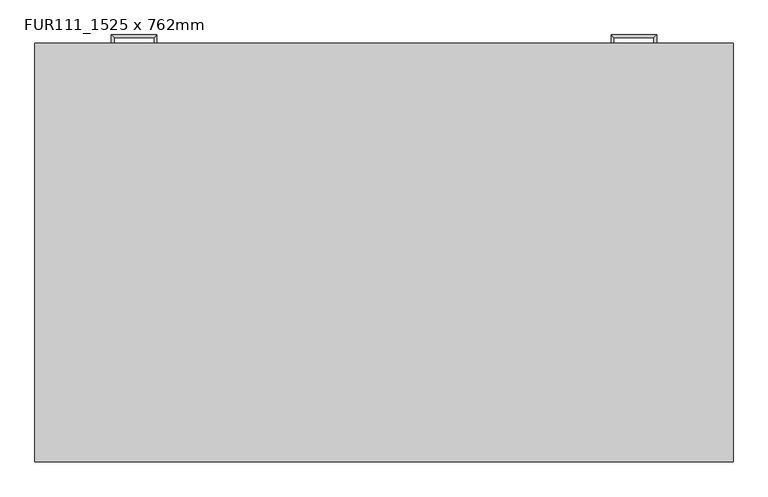
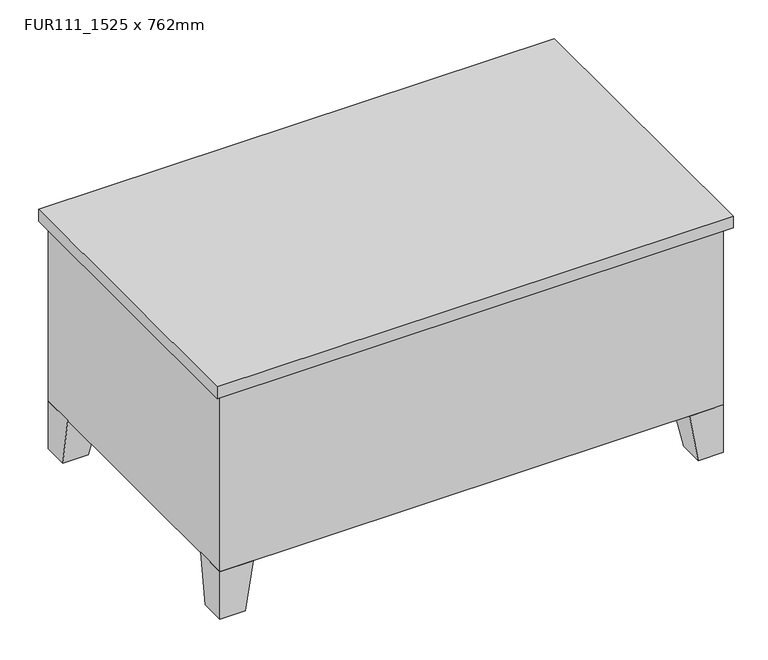
"""IFC4 building model written with IfcOpenShell, lengths in millimetres: furniture geometry, 책상 : FUR111_1525 x 762mm."""

from ifc_helpers import new_model, si_unit, frame, origin, place, context, project, spatial, polyline, outline, extrude, faceted_brep, source, transform, mapped, element, save


def fur111_1525_x_762mm_85151d33(model_context):
    return source(origin(), model_context, "Body", "SolidModel", [
        extrude(outline(polyline([(1505.95, 900.0), (1137.65, 900.0), (1137.65, 912.7), (1505.95, 912.7), (1505.95, 900.0)])), frame((0.0, 0.0, 603.25), z_axis=(0.0, 0.0, 1.0), x_axis=(1.0, 0.0, 0.0)), (0.0, 0.0, 1.0), 101.6),
        extrude(outline(polyline([(1505.95, 900.0), (1137.65, 900.0), (1137.65, 912.7), (1505.95, 912.7), (1505.95, 900.0)])), frame((0.0, 0.0, 171.05), z_axis=(0.0, 0.0, 1.0), x_axis=(1.0, 0.0, 0.0)), (0.0, 0.0, 1.0), 413.15),
        extrude(outline(polyline([(387.35, 900.0), (19.05, 900.0), (19.05, 912.7), (387.35, 912.7), (387.35, 900.0)])), frame((0.0, 0.0, 602.85), z_axis=(0.0, 0.0, 1.0), x_axis=(1.0, 0.0, 0.0)), (0.0, 0.0, 1.0), 102.0),
        extrude(outline(polyline([(387.35, 900.0), (19.05, 900.0), (19.05, 912.7), (387.35, 912.7), (387.35, 900.0)])), frame((0.0, 0.0, 171.05), z_axis=(0.0, 0.0, 1.0), x_axis=(1.0, 0.0, 0.0)), (0.0, 0.0, 1.0), 171.45),
        extrude(outline(polyline([(387.35, 900.0), (19.05, 900.0), (19.05, 912.7), (387.35, 912.7), (387.35, 900.0)])), frame((0.0, 0.0, 482.2), z_axis=(0.0, 0.0, 1.0), x_axis=(1.0, 0.0, 0.0)), (0.0, 0.0, 1.0), 101.6),
        extrude(outline(polyline([(387.35, 900.0), (19.05, 900.0), (19.05, 912.7), (387.35, 912.7), (387.35, 900.0)])), frame((0.0, 0.0, 361.55), z_axis=(0.0, 0.0, 1.0), x_axis=(1.0, 0.0, 0.0)), (0.0, 0.0, 1.0), 101.6),
        faceted_brep([(1423.4, 900.0, 152.0), (1423.4, 798.4, 152.0), (1525.0, 798.4, 152.0), (1525.0, 900.0, 152.0), (1448.8, 900.0, 0.0), (1525.0, 900.0, 0.0), (1525.0, 823.8, 0.0), (1448.8, 823.8, 0.0)], [[[0, 1, 2, 3]], [[4, 5, 6, 7]], [[4, 7, 1, 0]], [[7, 6, 2, 1]], [[6, 5, 3, 2]], [[5, 4, 0, 3]]]),
        faceted_brep([(1423.4, 0.0, 152.0), (1525.0, 0.0, 152.0), (1525.0, 101.6, 152.0), (1423.4, 101.6, 152.0), (1448.8, 0.0, 0.0), (1448.8, 76.2, 0.0), (1525.0, 76.2, 0.0), (1525.0, 0.0, 0.0)], [[[0, 1, 2, 3]], [[4, 5, 6, 7]], [[4, 7, 1, 0]], [[7, 6, 2, 1]], [[6, 5, 3, 2]], [[5, 4, 0, 3]]]),
        faceted_brep([(101.6, 0.0, 152.0), (101.6, 101.6, 152.0), (0.0, 101.6, 152.0), (0.0, 0.0, 152.0), (76.2, 0.0, 0.0), (0.0, 0.0, 0.0), (0.0, 76.2, 0.0), (76.2, 76.2, 0.0)], [[[0, 1, 2, 3]], [[4, 5, 6, 7]], [[4, 7, 1, 0]], [[7, 6, 2, 1]], [[6, 5, 3, 2]], [[5, 4, 0, 3]]]),
        faceted_brep([(101.6, 900.0, 152.0), (0.0, 900.0, 152.0), (0.0, 798.4, 152.0), (101.6, 798.4, 152.0), (76.2, 900.0, 0.0), (76.2, 823.8, 0.0), (0.0, 823.8, 0.0), (0.0, 900.0, 0.0)], [[[0, 1, 2, 3]], [[4, 5, 6, 7]], [[4, 7, 1, 0]], [[7, 6, 2, 1]], [[6, 5, 3, 2]], [[5, 4, 0, 3]]]),
        extrude(outline(polyline([(1544.05, 919.05), (1544.05, -19.05), (-19.05, -19.05), (-19.05, 919.05), (1544.05, 919.05)])), frame((0.0, 0.0, 723.9), z_axis=(0.0, 0.0, 1.0), x_axis=(1.0, 0.0, 0.0)), (0.0, 0.0, 1.0), 38.1),
        extrude(outline(polyline([(406.4, 900.0), (406.4, 50.8), (1118.6, 50.8), (1118.6, 900.0), (1525.0, 900.0), (1525.0, 0.0), (0.0, 0.0), (0.0, 900.0), (406.4, 900.0)])), frame((0.0, 0.0, 152.0), z_axis=(0.0, 0.0, 1.0), x_axis=(1.0, 0.0, 0.0)), (0.0, 0.0, 1.0), 571.9),
        faceted_brep([(1366.25, 912.7, 546.1), (1366.25, 912.7, 533.4), (1372.6, 912.7, 533.4), (1372.6, 912.7, 546.1), (1366.25, 931.75, 546.1), (1366.25, 931.75, 533.4), (1372.6, 938.1, 533.4), (1372.6, 938.1, 546.1), (1277.35, 931.75, 546.1), (1277.35, 931.75, 533.4), (1271.0, 938.1, 533.4), (1271.0, 938.1, 546.1), (1277.35, 912.7, 546.1), (1271.0, 912.7, 546.1), (1271.0, 912.7, 533.4), (1277.35, 912.7, 533.4)], [[[0, 1, 2, 3]], [[1, 0, 4, 5]], [[2, 1, 5, 6]], [[3, 2, 6, 7]], [[0, 3, 7, 4]], [[5, 4, 8, 9]], [[6, 5, 9, 10]], [[7, 6, 10, 11]], [[4, 7, 11, 8]], [[12, 13, 14, 15]], [[9, 8, 12, 15]], [[10, 9, 15, 14]], [[11, 10, 14, 13]], [[8, 11, 13, 12]]]),
        faceted_brep([(1366.25, 912.7, 666.75), (1366.25, 912.7, 654.05), (1372.6, 912.7, 654.05), (1372.6, 912.7, 666.75), (1366.25, 931.75, 666.75), (1366.25, 931.75, 654.05), (1372.6, 938.1, 654.05), (1372.6, 938.1, 666.75), (1277.35, 931.75, 666.75), (1277.35, 931.75, 654.05), (1271.0, 938.1, 654.05), (1271.0, 938.1, 666.75), (1277.35, 912.7, 666.75), (1271.0, 912.7, 666.75), (1271.0, 912.7, 654.05), (1277.35, 912.7, 654.05)], [[[0, 1, 2, 3]], [[1, 0, 4, 5]], [[2, 1, 5, 6]], [[3, 2, 6, 7]], [[0, 3, 7, 4]], [[5, 4, 8, 9]], [[6, 5, 9, 10]], [[7, 6, 10, 11]], [[4, 7, 11, 8]], [[12, 13, 14, 15]], [[9, 8, 12, 15]], [[10, 9, 15, 14]], [[11, 10, 14, 13]], [[8, 11, 13, 12]]]),
        faceted_brep([(158.75, 912.7, 304.8), (152.4, 912.7, 304.8), (152.4, 912.7, 292.1), (158.75, 912.7, 292.1), (158.75, 931.75, 304.8), (152.4, 938.1, 304.8), (152.4, 938.1, 292.1), (158.75, 931.75, 292.1), (247.65, 931.75, 304.8), (254.0, 938.1, 304.8), (254.0, 938.1, 292.1), (247.65, 931.75, 292.1), (247.65, 912.7, 304.8), (247.65, 912.7, 292.1), (254.0, 912.7, 292.1), (254.0, 912.7, 304.8)], [[[0, 1, 2, 3]], [[1, 0, 4, 5]], [[2, 1, 5, 6]], [[3, 2, 6, 7]], [[0, 3, 7, 4]], [[5, 4, 8, 9]], [[6, 5, 9, 10]], [[7, 6, 10, 11]], [[4, 7, 11, 8]], [[12, 13, 14, 15]], [[9, 8, 12, 15]], [[10, 9, 15, 14]], [[11, 10, 14, 13]], [[8, 11, 13, 12]]]),
        faceted_brep([(158.75, 912.7, 425.45), (152.4, 912.7, 425.45), (152.4, 912.7, 412.75), (158.75, 912.7, 412.75), (158.75, 931.75, 425.45), (152.4, 938.1, 425.45), (152.4, 938.1, 412.75), (158.75, 931.75, 412.75), (247.65, 931.75, 425.45), (254.0, 938.1, 425.45), (254.0, 938.1, 412.75), (247.65, 931.75, 412.75), (247.65, 912.7, 425.45), (247.65, 912.7, 412.75), (254.0, 912.7, 412.75), (254.0, 912.7, 425.45)], [[[0, 1, 2, 3]], [[1, 0, 4, 5]], [[2, 1, 5, 6]], [[3, 2, 6, 7]], [[0, 3, 7, 4]], [[5, 4, 8, 9]], [[6, 5, 9, 10]], [[7, 6, 10, 11]], [[4, 7, 11, 8]], [[12, 13, 14, 15]], [[9, 8, 12, 15]], [[10, 9, 15, 14]], [[11, 10, 14, 13]], [[8, 11, 13, 12]]]),
        faceted_brep([(158.75, 912.7, 546.1), (152.4, 912.7, 546.1), (152.4, 912.7, 533.4), (158.75, 912.7, 533.4), (158.75, 931.75, 546.1), (152.4, 938.1, 546.1), (152.4, 938.1, 533.4), (158.75, 931.75, 533.4), (247.65, 931.75, 546.1), (254.0, 938.1, 546.1), (254.0, 938.1, 533.4), (247.65, 931.75, 533.4), (247.65, 912.7, 546.1), (247.65, 912.7, 533.4), (254.0, 912.7, 533.4), (254.0, 912.7, 546.1)], [[[0, 1, 2, 3]], [[1, 0, 4, 5]], [[2, 1, 5, 6]], [[3, 2, 6, 7]], [[0, 3, 7, 4]], [[5, 4, 8, 9]], [[6, 5, 9, 10]], [[7, 6, 10, 11]], [[4, 7, 11, 8]], [[12, 13, 14, 15]], [[9, 8, 12, 15]], [[10, 9, 15, 14]], [[11, 10, 14, 13]], [[8, 11, 13, 12]]]),
        faceted_brep([(158.75, 912.7, 666.75), (152.4, 912.7, 666.75), (152.4, 912.7, 654.05), (158.75, 912.7, 654.05), (158.75, 931.75, 666.75), (152.4, 938.1, 666.75), (152.4, 938.1, 654.05), (158.75, 931.75, 654.05), (247.65, 931.75, 666.75), (254.0, 938.1, 666.75), (254.0, 938.1, 654.05), (247.65, 931.75, 654.05), (247.65, 912.7, 666.75), (247.65, 912.7, 654.05), (254.0, 912.7, 654.05), (254.0, 912.7, 666.75)], [[[0, 1, 2, 3]], [[1, 0, 4, 5]], [[2, 1, 5, 6]], [[3, 2, 6, 7]], [[0, 3, 7, 4]], [[5, 4, 8, 9]], [[6, 5, 9, 10]], [[7, 6, 10, 11]], [[4, 7, 11, 8]], [[12, 13, 14, 15]], [[9, 8, 12, 15]], [[10, 9, 15, 14]], [[11, 10, 14, 13]], [[8, 11, 13, 12]]]),
    ])


if __name__ == "__main__":
    model = new_model("IFC4")
    model_context = context("Model", 3, world=origin())
    ifc_project = project(units=[si_unit("LENGTHUNIT", "METRE", prefix="MILLI")], contexts=[model_context])
    site = spatial("IfcSite", under=ifc_project)
    building = spatial("IfcBuilding", under=site)
    placement = place(None, origin())
    fur111_1525_x_762mm_shape = fur111_1525_x_762mm_85151d33(model_context)
    element("IfcFurniture", 1, ObjectType="책상 : FUR111_1525 x 762mm", at=placement, inside=building, context=model_context, shape_type="MappedRepresentation", body=[
        mapped(fur111_1525_x_762mm_shape, transform((0.0, 0.0, 0.0), x_axis=(1.0, 0.0, 0.0), y_axis=(0.0, 1.0, 0.0), z_axis=(0.0, 0.0, 1.0))),
    ])
    save(model, "model.ifc")

# Revit data of these elements
# Type "책상 : FUR111_1525 x 762mm"
#   깊이 = 900 mm
#   높이 = 762 mm
#   다리 높이 = 152 mm
#   폭 = 1525 mm
#   본체 재료 = 라미네이티드 플라스틱 - 아이보리색, 무광
#   핸들/다리 재료 = 금속 - 크롬
#   상단 재료 = 목재 - 벚나무
#   Default Elevation = 0
# Element 1 (IfcFurniture, "책상 : FUR111_1525 x 762mm")
#   Materials on its faces: "금속 - 크롬", "라미네이티드 플라스틱 - 아이보리색, 무광", "목재 - 벚나무"
# Materials
#   "라미네이티드 플라스틱 - 아이보리색, 무광": class "다양한", colour RGB 247 247 239, transparency 0
#   "금속 - 크롬": class "금속", colour RGB 17 17 17, transparency 0
#   "목재 - 벚나무": class "목재", colour RGB 226 177 128, transparency 0
